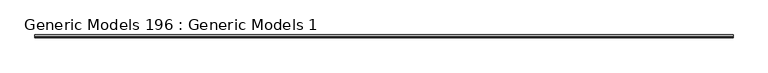
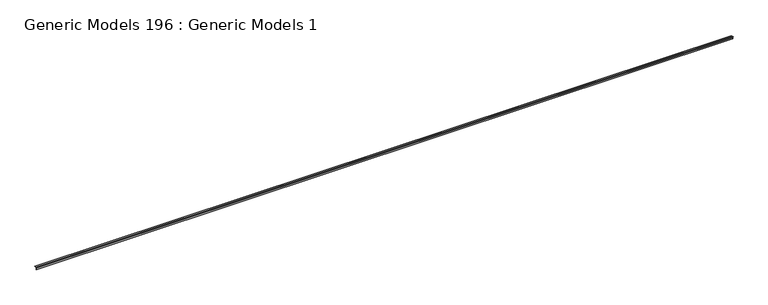
"""IFC4 building model written with IfcOpenShell, lengths in millimetres: proxy geometry, Generic Models 196 : Generic Models 1."""

from ifc_helpers import new_model, si_unit, point, frame, frame_2d, origin, place, context, project, spatial, polyline, circle_curve, trimmed, segment, composite_curve, outline, extrude, source, transform, mapped, element, save


def generic_models_196_generic_models_1_f1e25639(model_context):
    return source(origin(), model_context, "Body", "SweptSolid", [
        extrude(outline(composite_curve([segment(polyline([(-25410.3679897, 127166.5926156), (-25372.3424751, 127147.066), (-25334.2424751, 127147.066), (-25334.2424751, 127145.796), (-25372.6494989, 127145.796), (-25411.4025971, 127165.6962396), (-25391.5023575, 127126.9431414), (-25391.5023575, 127088.5361176), (-25392.7723575, 127088.5361176), (-25392.7723575, 127126.6361176), (-25412.2989731, 127164.6616323)]), True, "CONTINUOUS"), segment(trimmed(circle_curve(frame_2d((-25411.0231448, 127165.3167873)), 1.4342127), [point((-25412.2989731, 127164.6616323))], [point((-25410.3679897, 127166.5926156))], False, "CARTESIAN"), True, "CONTINUOUS")], self_intersect=False)), frame((-20998.9733045, 0.0, 0.0), z_axis=(1.0, 0.0, 0.0), x_axis=(0.0, 1.0, 0.0)), (0.0, 0.0, 1.0), 19050.0),
    ])


if __name__ == "__main__":
    model = new_model("IFC4")
    model_context = context("Model", 3, world=origin())
    ifc_project = project(units=[si_unit("LENGTHUNIT", "METRE", prefix="MILLI")], contexts=[model_context])
    site = spatial("IfcSite", under=ifc_project)
    building = spatial("IfcBuilding", under=site)
    placement = place(None, origin())
    generic_models_196_generic_models_1_shape = generic_models_196_generic_models_1_f1e25639(model_context)
    element("IfcBuildingElementProxy", 1, Name="Generic Models 196 : Generic Models 1", ObjectType="Generic Models 196 : Generic Models 1", at=placement, inside=building, context=model_context, shape_type="MappedRepresentation", body=[
        mapped(generic_models_196_generic_models_1_shape, transform((0.0, 0.0, 0.0), x_axis=(1.0, 0.0, 0.0), y_axis=(0.0, 1.0, 0.0), z_axis=(0.0, 0.0, 1.0))),
    ])
    save(model, "model.ifc")

# Revit data of these elements
# Element 1 (IfcBuildingElementProxy, "Generic Models 196 : Generic Models 1")
#   Materials on its faces: "_CONTINIOUS 16 GA. COPPER CORNER BEAD"
# Materials
#   "_CONTINIOUS 16 GA. COPPER CORNER BEAD": class "Generic", colour RGB 253 192 103, transparency 0, Cost = 0
